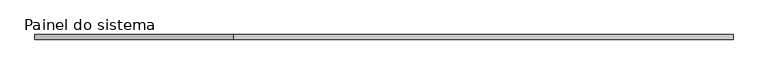
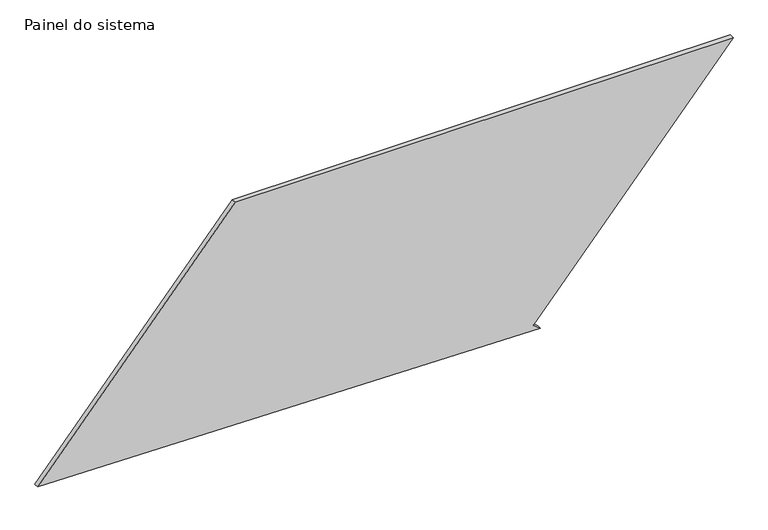
"""IFC4 building model written with IfcOpenShell, lengths in millimetres: plate geometry, Painel do sistema : Envidraçado."""

from ifc_helpers import new_model, si_unit, frame, origin, place, context, project, spatial, polyline, outline, extrude, source, transform, mapped, element, save


def painel_do_sistema_65ef20ba(model_context):
    return source(origin(), model_context, "Body", "SweptSolid", [
        extrude(outline(polyline([(0.0, 843.903653), (32.4485234, 805.8629731), (1306.0982198, 1892.2802547), (1306.0982198, -817.7860487), (46.4264139, -1892.2802547), (0.0, 843.903653)])), frame((0.0, 24.5, 0.0), z_axis=(0.0, 1.0, 0.0), x_axis=(0.0, 0.0, 1.0)), (0.0, 0.0, 1.0), 25.0),
    ])


if __name__ == "__main__":
    model = new_model("IFC4")
    model_context = context("Model", 3, world=origin())
    ifc_project = project(units=[si_unit("LENGTHUNIT", "METRE", prefix="MILLI")], contexts=[model_context])
    site = spatial("IfcSite", under=ifc_project)
    building = spatial("IfcBuilding", under=site)
    placement = place(None, origin())
    painel_do_sistema_shape = painel_do_sistema_65ef20ba(model_context)
    element("IfcPlate", 1, ObjectType="Painel do sistema : Envidraçado", at=placement, inside=building, context=model_context, shape_type="MappedRepresentation", body=[
        mapped(painel_do_sistema_shape, transform((0.0, 0.0, 0.0), x_axis=(1.0, 0.0, 0.0), y_axis=(0.0, 1.0, 0.0), z_axis=(0.0, 0.0, 1.0))),
    ])
    save(model, "model.ifc")

# Revit data of these elements
# Type "Painel do sistema : Envidraçado"
#   Construction Type Id = "GSP4R"
#   Analytic Construction = "Vidraça única Pilkington 1/8 pol"
#   Visual Light Transmittance = 0.9
#   Solar Heat Gain Coefficient = 0.86
#   Heat Transfer Coefficient (U) = 6.7069 W/(m²·K)
# Element 1 (IfcPlate, "Painel do sistema : Envidraçado")
#   Materials on its faces: "Vidro"
# Materials
#   "Vidro": class "Vidro", colour RGB 0 128 192, transparency 0.9, Description = "Vidro de sílica", Cost = 0
